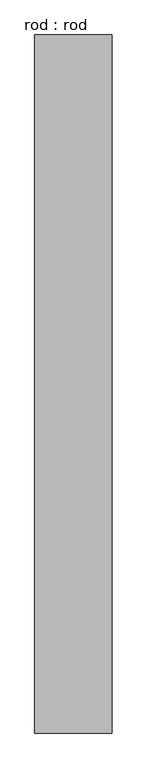
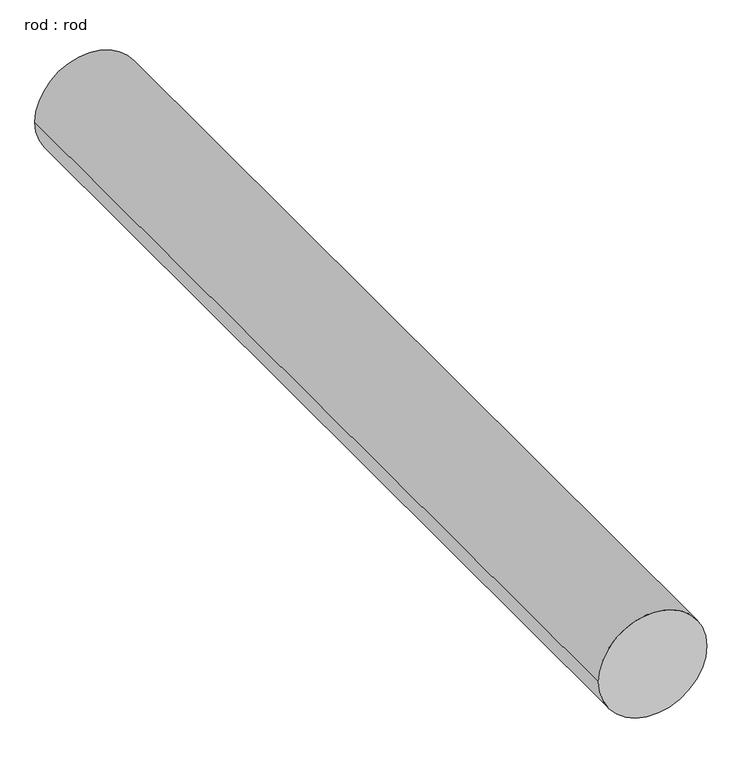
"""IFC4 building model written with IfcOpenShell, lengths in millimetres: proxy geometry, rod : rod."""

from ifc_helpers import new_model, si_unit, point, frame, frame_2d, origin, place, context, project, spatial, circle_curve, trimmed, segment, composite_curve, outline, extrude, source, transform, mapped, element, save


def rod_rod_6c0f80b8(model_context):
    return source(origin(), model_context, "Body", "SweptSolid", [
        extrude(outline(composite_curve([segment(trimmed(circle_curve(frame_2d((0.0108462, 0.0)), 200.0), [point((0.0108462, 200.0))], [point((0.0108462, -200.0))], False, "CARTESIAN"), True, "CONTINUOUS"), segment(trimmed(circle_curve(frame_2d((0.0108462, 0.0)), 200.0), [point((0.0108462, -200.0))], [point((0.0108462, 200.0))], False, "CARTESIAN"), True, "CONTINUOUS")], self_intersect=False)), frame((0.0, 2290.9083552, 0.0), z_axis=(0.0, 1.0, 0.0), x_axis=(0.0, 0.0, 1.0)), (0.0, 0.0, 1.0), 3603.6405204),
    ])


if __name__ == "__main__":
    model = new_model("IFC4")
    model_context = context("Model", 3, world=origin())
    ifc_project = project(units=[si_unit("LENGTHUNIT", "METRE", prefix="MILLI")], contexts=[model_context])
    site = spatial("IfcSite", under=ifc_project)
    building = spatial("IfcBuilding", under=site)
    placement = place(None, origin())
    rod_rod_shape = rod_rod_6c0f80b8(model_context)
    element("IfcBuildingElementProxy", 1, Name="rod : rod", ObjectType="rod : rod", at=placement, inside=building, context=model_context, shape_type="MappedRepresentation", body=[
        mapped(rod_rod_shape, transform((0.0, 0.0, 0.0), x_axis=(1.0, 0.0, 0.0), y_axis=(0.0, 1.0, 0.0), z_axis=(0.0, 0.0, 1.0))),
    ])
    save(model, "model.ifc")

# Revit data of these elements
# Type "rod : rod"
#   Default Elevation = 0
